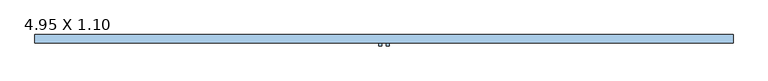
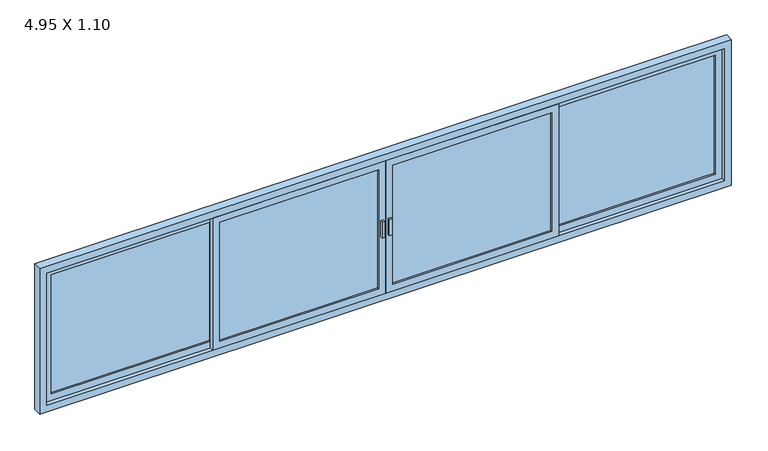
"""IFC4 building model written with IfcOpenShell, lengths in millimetres: window geometry, .CC_ND 300_JANELA_4 FOLHAS DE CORRER_VIDRO : 4.95 X 1.10."""

from ifc_helpers import new_model, si_unit, frame, origin, place, context, project, spatial, polyline, outline, extrude, source, transform, mapped, element, save


def window_4_95_x_1_10_4a8d5465(model_context):
    return source(origin(), model_context, "Body", "SweptSolid", [
        extrude(outline(polyline([(-50.0, -12.5), (-50.0, -17.5), (-1187.5, -17.5), (-1187.5, -12.5), (-50.0, -12.5)])), frame((0.0, 0.0, 1100.0), z_axis=(0.0, 0.0, 1.0), x_axis=(1.0, 0.0, 0.0)), (0.0, 0.0, 1.0), 900.0),
        extrude(outline(polyline([(2050.0, 0.0), (2050.0, -1237.5), (1050.0, -1237.5), (1050.0, 0.0), (2050.0, 0.0)]), holes=[polyline([(2000.0, -50.0), (1100.0, -50.0), (1100.0, -1187.5), (2000.0, -1187.5), (2000.0, -50.0)])]), frame((0.0, -30.0, 0.0), z_axis=(0.0, 1.0, 0.0), x_axis=(0.0, 0.0, 1.0)), (0.0, 0.0, 1.0), 30.0),
        extrude(outline(polyline([(-1237.5, 17.5), (-1237.5, 12.5), (-2375.0, 12.5), (-2375.0, 17.5), (-1237.5, 17.5)])), frame((0.0, 0.0, 1100.0), z_axis=(0.0, 0.0, 1.0), x_axis=(1.0, 0.0, 0.0)), (0.0, 0.0, 1.0), 900.0),
        extrude(outline(polyline([(2050.0, -1187.5), (2050.0, -2425.0), (1050.0, -2425.0), (1050.0, -1187.5), (2050.0, -1187.5)]), holes=[polyline([(2000.0, -1237.5), (1100.0, -1237.5), (1100.0, -2375.0), (2000.0, -2375.0), (2000.0, -1237.5)])]), frame((0.0, 0.0, 0.0), z_axis=(0.0, 1.0, 0.0), x_axis=(0.0, 0.0, 1.0)), (0.0, 0.0, 1.0), 30.0),
        extrude(outline(polyline([(2375.0, 17.5), (2375.0, 12.5), (1237.5, 12.5), (1237.5, 17.5), (2375.0, 17.5)])), frame((0.0, 0.0, 1100.0), z_axis=(0.0, 0.0, 1.0), x_axis=(1.0, 0.0, 0.0)), (0.0, 0.0, 1.0), 900.0),
        extrude(outline(polyline([(2050.0, 2425.0), (2050.0, 1187.5), (1050.0, 1187.5), (1050.0, 2425.0), (2050.0, 2425.0)]), holes=[polyline([(2000.0, 2375.0), (1100.0, 2375.0), (1100.0, 1237.5), (2000.0, 1237.5), (2000.0, 2375.0)])]), frame((0.0, 0.0, 0.0), z_axis=(0.0, 1.0, 0.0), x_axis=(0.0, 0.0, 1.0)), (0.0, 0.0, 1.0), 30.0),
        extrude(outline(polyline([(1187.5, -12.5), (1187.5, -17.5), (50.0, -17.5), (50.0, -12.5), (1187.5, -12.5)])), frame((0.0, 0.0, 1100.0), z_axis=(0.0, 0.0, 1.0), x_axis=(1.0, 0.0, 0.0)), (0.0, 0.0, 1.0), 900.0),
        extrude(outline(polyline([(2050.0, 1237.5), (2050.0, 0.0), (1050.0, 0.0), (1050.0, 1237.5), (2050.0, 1237.5)]), holes=[polyline([(2000.0, 1187.5), (1100.0, 1187.5), (1100.0, 50.0), (2000.0, 50.0), (2000.0, 1187.5)])]), frame((0.0, -30.0, 0.0), z_axis=(0.0, 1.0, 0.0), x_axis=(0.0, 0.0, 1.0)), (0.0, 0.0, 1.0), 30.0),
        extrude(outline(polyline([(1000.0, -2475.0), (1000.0, 2475.0), (2100.0, 2475.0), (2100.0, -2475.0), (1000.0, -2475.0)]), holes=[polyline([(2050.0, -2425.0), (2050.0, 2425.0), (1050.0, 2425.0), (1050.0, -2425.0), (2050.0, -2425.0)])]), frame((0.0, -30.0, 0.0), z_axis=(0.0, 1.0, 0.0), x_axis=(0.0, 0.0, 1.0)), (0.0, 0.0, 1.0), 60.0),
        extrude(outline(polyline([(-35.9492003, -30.0), (-15.9492003, -30.0), (-15.9492003, -50.0), (-35.9492003, -50.0), (-35.9492003, -30.0)])), frame((0.0, 0.0, 1490.0), z_axis=(0.0, 0.0, 1.0), x_axis=(1.0, 0.0, 0.0)), (0.0, 0.0, 1.0), 120.0),
        extrude(outline(polyline([(15.9492003, -30.0), (35.9492003, -30.0), (35.9492003, -50.0), (15.9492003, -50.0), (15.9492003, -30.0)])), frame((0.0, 0.0, 1490.0), z_axis=(0.0, 0.0, 1.0), x_axis=(1.0, 0.0, 0.0)), (0.0, 0.0, 1.0), 120.0),
    ])


if __name__ == "__main__":
    model = new_model("IFC4")
    model_context = context("Model", 3, world=origin())
    ifc_project = project(units=[si_unit("LENGTHUNIT", "METRE", prefix="MILLI")], contexts=[model_context])
    site = spatial("IfcSite", under=ifc_project)
    building = spatial("IfcBuilding", under=site)
    placement = place(None, origin())
    window_4_95_x_1_10_shape = window_4_95_x_1_10_4a8d5465(model_context)
    element("IfcWindow", 1, ObjectType=".CC_ND 300_JANELA_4 FOLHAS DE CORRER_VIDRO : 4.95 X 1.10", at=placement, inside=building, context=model_context, shape_type="MappedRepresentation", body=[
        mapped(window_4_95_x_1_10_shape, transform((0.0, 0.0, 0.0), x_axis=(1.0, 0.0, 0.0), y_axis=(0.0, 1.0, 0.0), z_axis=(0.0, 0.0, 1.0))),
    ])
    save(model, "model.ifc")

# Revit data of these elements
# Type ".CC_ND 300_JANELA_4 FOLHAS DE CORRER_VIDRO : 4.95 X 1.10"
#   Type Mark = "69"
#   Largura moldura = 0.06 m
#   Largura janela = 4.85 m
#   Largura esquadria = 0.05 m
#   Largura do painel = 1.2375 m
#   Largura da moldura do painel = 0.05 m
#   Espessura painel = 0.03 m
#   Espessura moldura = 0.03 m
#   Altura janela = 1.00 m
#   Height = 1.10 m
#   Altura-padrão do peitoril = 1.00 m
#   Width = 4.95 m
#   Puxadores [instance default] = yes
#   Moldura interna [instance default] = yes
#   Moldura externa [instance default] = yes
#   Tipo de vidro = .VIDRO GENÉRICO
#   Material puxadores = .ALUMÍNIO COM PINTURA ELETROSTÁTICA BRANCA
#   Material moldura = .ALUMÍNIO COM PINTURA ELETROSTÁTICA BRANCA
#   Material da esquadria = .ALUMÍNIO COM PINTURA ELETROSTÁTICA BRANCA
#   Wall Closure = (empty or 0)
# Element 1 (IfcWindow, ".CC_ND 300_JANELA_4 FOLHAS DE CORRER_VIDRO : 4.95 X 1.10")
#   Moldura interna = no
#   Moldura externa = no
#   Materials on its faces: ".ALUMÍNIO COM PINTURA ELETROSTÁTICA BRANCA", ".VIDRO GENÉRICO"
# Materials
#   ".VIDRO GENÉRICO": class ".CC_VIDRO", colour RGB 0 128 192, transparency 0.9, Description = "Vidro comum", Cost = 0
#   ".ALUMÍNIO COM PINTURA ELETROSTÁTICA BRANCA": class "CC_METAIS", colour RGB 241 241 241, transparency 0, Cost = 0
